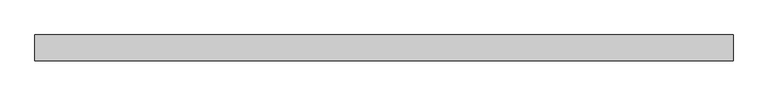
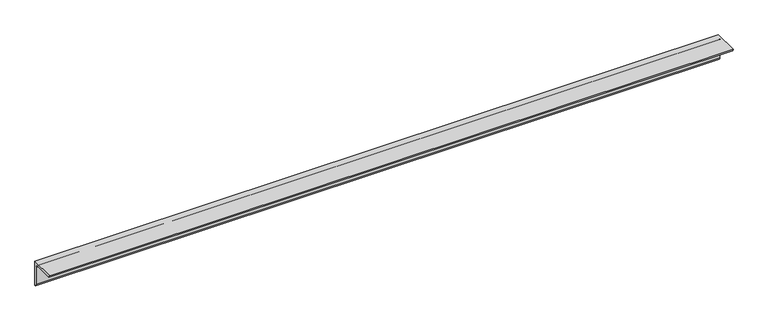
"""IFC4 building model written with IfcOpenShell, lengths in millimetres: member geometry, 0912_Steel Framing_L-KSD3502 : H_SB_AR_S03_L-130x130x12_HBR3."""

from ifc_helpers import new_model, si_unit, point, frame, frame_2d, origin, place, context, project, spatial, polyline, circle_curve, trimmed, segment, composite_curve, outline, extrude, source, transform, mapped, element, save


def member_599d3c72(model_context):
    return source(origin(), model_context, "Body", "SweptSolid", [
        extrude(outline(composite_curve([segment(polyline([(36.4, 36.4), (36.4, -93.6)]), True, "CONTINUOUS"), segment(trimmed(circle_curve(frame_2d((36.4, -81.6)), 12.0), [point((36.4, -93.6))], [point((24.4, -81.6))], False, "CARTESIAN"), True, "CONTINUOUS"), segment(polyline([(24.4, -81.6), (24.4, 12.4)]), True, "CONTINUOUS"), segment(trimmed(circle_curve(frame_2d((12.4, 12.4)), 12.0), [point((24.4, 12.4))], [point((12.4, 24.4))], True, "CARTESIAN"), True, "CONTINUOUS"), segment(polyline([(12.4, 24.4), (-81.6, 24.4)]), True, "CONTINUOUS"), segment(trimmed(circle_curve(frame_2d((-81.6, 36.4)), 12.0), [point((-81.6, 24.4))], [point((-93.6, 36.4))], False, "CARTESIAN"), True, "CONTINUOUS"), segment(polyline([(-93.6, 36.4), (36.4, 36.4)]), True, "CONTINUOUS")], self_intersect=False)), frame((-1742.0220284, 0.0, 0.0), z_axis=(1.0, 0.0, 0.0), x_axis=(0.0, 1.0, 0.0)), (0.0, 0.0, 1.0), 3516.2103492),
    ])


if __name__ == "__main__":
    model = new_model("IFC4")
    model_context = context("Model", 3, world=origin())
    ifc_project = project(units=[si_unit("LENGTHUNIT", "METRE", prefix="MILLI")], contexts=[model_context])
    site = spatial("IfcSite", under=ifc_project)
    building = spatial("IfcBuilding", under=site)
    placement = place(None, origin())
    member_shape = member_599d3c72(model_context)
    element("IfcMember", 1, ObjectType="0912_Steel Framing_L-KSD3502 : H_SB_AR_S03_L-130x130x12_HBR3", at=placement, inside=building, context=model_context, shape_type="MappedRepresentation", body=[
        mapped(member_shape, transform((0.0, 0.0, 0.0), x_axis=(1.0, 0.0, 0.0), y_axis=(0.0, 1.0, 0.0), z_axis=(0.0, 0.0, 1.0))),
    ])
    save(model, "model.ifc")

# Revit data of these elements
# Type "0912_Steel Framing_L-KSD3502 : H_SB_AR_S03_L-130x130x12_HBR3"
#   k = 25 mm
#   Perimeter = 0.52 m²/m
#   Nominal Weight = 23.40 kgf/m
#   Length [instance default] = 1000 mm
#   b = 130 mm
#   d = 130 mm
#   t = 12 mm
#   x = 36.4 mm
#   y = 36.4 mm
#   A = 2976.00 m²
#   Structural Material [instance default] = Steel, 45-345
# Element 1 (IfcMember, "0912_Steel Framing_L-KSD3502 : H_SB_AR_S03_L-130x130x12_HBR3")
#   Structural Material = Steel ASTM A36
#   Materials on its faces: "Steel ASTM A36"
# Materials
#   "Steel, 45-345": class "Metal", colour RGB 189 187 185, transparency 0, Description = "Steel 345 MPa", Cost = 0
#   "Steel ASTM A36": class "Metal", colour RGB 199 199 199, transparency 0, Description = "Structural steel, ASTM A36 Grade B, mill finish", Cost = 0
